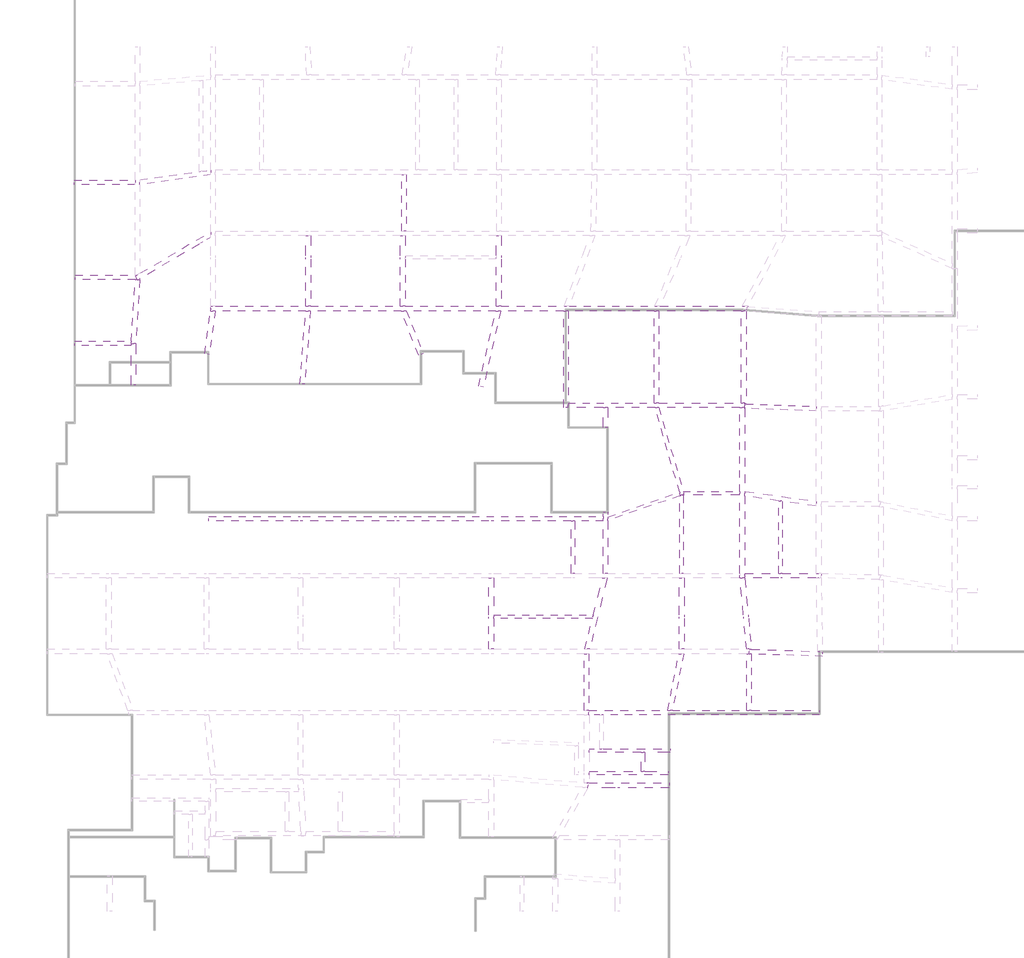
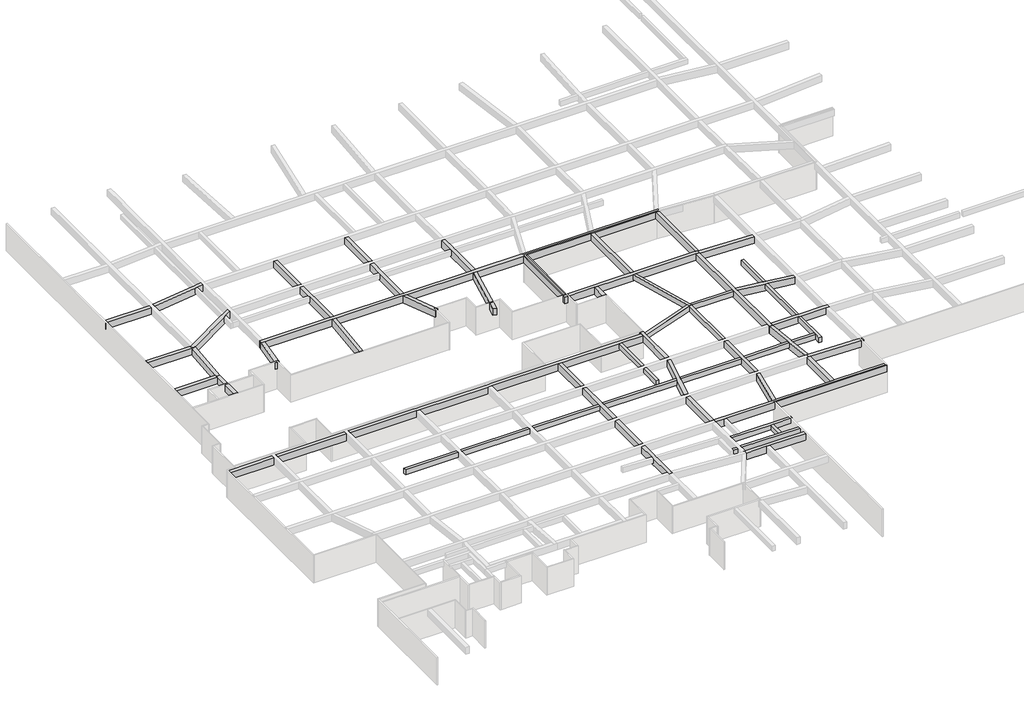
# One storey, part 7 of 16: 47 beams.
"""IFC4 building model written with IfcOpenShell, lengths in millimetres."""

from ifc_helpers import new_model, si_unit, frame, origin, place, context, project, spatial, polyline, outline, extrude, faceted_brep, element, save

model = new_model("IFC4")

# Units and contexts
model_context = context("Model", 3, world=origin())
ifc_project = project(units=[si_unit("LENGTHUNIT", "METRE", prefix="MILLI")], contexts=[model_context])

# Site, building, storey
site = spatial("IfcSite", under=ifc_project)
building = spatial("IfcBuilding", under=site)
storey = spatial("IfcBuildingStorey", under=building, Name="户型图", Elevation=0.0)

# Beams
placement = place(None, origin())
element("IfcBeam", 1, ObjectType="混凝土 - 矩形梁 : KL_beam", at=placement, inside=storey, context=model_context, shape_type="Brep", body=[
    faceted_brep([(78176.3134091, 116076.7662248, 3300.0), (78176.3134091, 115889.7208044, 3300.0), (78176.3134091, 115676.7662248, 3300.0), (78551.9803713, 115676.7662248, 3300.0), (86260.0613272, 115676.7662248, 3300.0), (86661.2679399, 115676.7662248, 3300.0), (94380.6776719, 115676.7662248, 3300.0), (94811.3414742, 115676.7662248, 3300.0), (102431.6143421, 115676.7662248, 3300.0), (102841.8811164, 115676.7662248, 3300.0), (108192.7086168, 115676.7662248, 3300.0), (108592.7086168, 115676.7662248, 3300.0), (115895.8554474, 115676.7662248, 3300.0), (116295.8554474, 115676.7662248, 3300.0), (123316.4637871, 115676.7662248, 3300.0), (123636.1686236, 115676.7662248, 3300.0), (123716.4637871, 115826.5354155, 3300.0), (123838.7967449, 116054.7148883, 3300.0), (123850.6190407, 116076.7662248, 3300.0), (123396.7589506, 116076.7662248, 3300.0), (116398.0224861, 116076.7662248, 3300.0), (115963.4783352, 116076.7662248, 3300.0), (108678.3382182, 116076.7662248, 3300.0), (108252.6671092, 116076.7662248, 3300.0), (102882.3515287, 116076.7662248, 3300.0), (102482.3515287, 116076.7662248, 3300.0), (94716.2109037, 116076.7662248, 3300.0), (94316.2109037, 116076.7662248, 3300.0), (86676.2109037, 116076.7662248, 3300.0), (86276.2109037, 116076.7662248, 3300.0), (78576.3134091, 116076.7662248, 3300.0), (78176.3134091, 115676.7662248, 2500.0), (78551.9803713, 115676.7662248, 2500.0), (86260.0613272, 115676.7662248, 2500.0), (86661.2679399, 115676.7662248, 2500.0), (94380.6776719, 115676.7662248, 2500.0), (94811.3414742, 115676.7662248, 2500.0), (102431.6143421, 115676.7662248, 2500.0), (102841.8811164, 115676.7662248, 2500.0), (108192.7086168, 115676.7662248, 2500.0), (108592.7086168, 115676.7662248, 2500.0), (115895.8554474, 115676.7662248, 2500.0), (116295.8554474, 115676.7662248, 2500.0), (123316.4637871, 115676.7662248, 2500.0), (123636.1686236, 115676.7662248, 2500.0), (78176.3134091, 115889.7208044, 2500.0), (78176.3134091, 116076.7662248, 2500.0), (78576.3134091, 116076.7662248, 2500.0), (86276.2109037, 116076.7662248, 2500.0), (86676.2109037, 116076.7662248, 2500.0), (94316.2109037, 116076.7662248, 2500.0), (94716.2109037, 116076.7662248, 2500.0), (102482.3515287, 116076.7662248, 2500.0), (102882.3515287, 116076.7662248, 2500.0), (108252.6671092, 116076.7662248, 2500.0), (108678.3382182, 116076.7662248, 2500.0), (115963.4783352, 116076.7662248, 2500.0), (116398.0224861, 116076.7662248, 2500.0), (123396.7589506, 116076.7662248, 2500.0), (123850.6190407, 116076.7662248, 2500.0), (123838.7967449, 116054.7148883, 2500.0), (123716.4637871, 115826.5354155, 2500.0)], [[[0, 1, 2, 3, 4, 5, 6, 7, 8, 9, 10, 11, 12, 13, 14, 15, 16, 17, 18, 19, 20, 21, 22, 23, 24, 25, 26, 27, 28, 29, 30]], [[2, 31, 32, 33, 34, 35, 36, 37, 38, 39, 40, 41, 42, 43, 44, 15, 14, 13, 12, 11, 10, 9, 8, 7, 6, 5, 4, 3]], [[31, 45, 46, 47, 48, 49, 50, 51, 52, 53, 54, 55, 56, 57, 58, 59, 60, 61, 44, 43, 42, 41, 40, 39, 38, 37, 36, 35, 34, 33, 32]], [[46, 0, 30, 29, 28, 27, 26, 25, 24, 23, 22, 21, 20, 19, 18, 59, 58, 57, 56, 55, 54, 53, 52, 51, 50, 49, 48, 47]], [[2, 1, 0, 46, 45, 31]], [[18, 17, 16, 15, 44, 61, 60, 59]]]),
])
element("IfcBeam", 2, ObjectType="混凝土 - 矩形梁 : KL_beam", at=placement, inside=storey, context=model_context, shape_type="SweptSolid", body=[
    extrude(outline(polyline([(78070.7151318, 111977.3325661), (77674.0575313, 112028.9343875), (78176.3134091, 115889.7208044), (78176.3134091, 115676.7662248), (78551.9803713, 115676.7662248), (78070.7151318, 111977.3325661)])), frame((0.0, 0.0, 2500.0), z_axis=(0.0, 0.0, 1.0), x_axis=(1.0, 0.0, 0.0)), (0.0, 0.0, 1.0), 800.0),
])
element("IfcBeam", 3, ObjectType="混凝土 - 矩形梁 : KL_beam", at=placement, inside=storey, context=model_context, shape_type="Brep", body=[
    faceted_brep([(86276.2109037, 116076.7662248, 3300.0), (86676.2109037, 116076.7662248, 3300.0), (86676.2109037, 120066.4564837, 3300.0), (86676.2109037, 120366.4564837, 3300.0), (86676.2109037, 122085.5220623, 3300.0), (86276.2109037, 122085.5220623, 3300.0), (86276.2109037, 120366.4564837, 3300.0), (86276.2109037, 120066.4564837, 3300.0), (86676.2109037, 116076.7662248, 2500.0), (86676.2109037, 122085.5220623, 2500.0), (86276.2109037, 116076.7662248, 2500.0), (86276.2109037, 122085.5220623, 2500.0)], [[[0, 1, 2, 3, 4, 5, 6, 7]], [[1, 8, 9, 4, 3, 2]], [[8, 10, 11, 9]], [[10, 0, 7, 6, 5, 11]], [[1, 0, 10, 8]], [[5, 4, 9, 11]]]),
    faceted_brep([(86276.2109037, 127293.5189202, 3300.0), (86676.2109037, 127293.5189202, 3300.0), (86676.2109037, 127293.5189202, 2500.0), (86276.2109037, 127293.5189202, 2500.0), (86676.2109037, 122485.5220623, 3300.0), (86276.2109037, 122485.5220623, 3300.0), (86276.2109037, 122485.5220623, 2500.0), (86676.2109037, 122485.5220623, 2500.0)], [[[0, 1, 2, 3]], [[4, 5, 6, 7]], [[1, 0, 5, 4]], [[2, 1, 4, 7]], [[3, 2, 7, 6]], [[0, 3, 6, 5]]]),
])
element("IfcBeam", 4, ObjectType="混凝土 - 矩形梁 : KL_beam", at=placement, inside=storey, context=model_context, shape_type="Brep", body=[
    faceted_brep([(102882.3515287, 122085.5220623, 3300.0), (102482.3515287, 122085.5220623, 3300.0), (102482.3515287, 120366.4564837, 3300.0), (102482.3515287, 120066.4564837, 3300.0), (102482.3515287, 116076.7662248, 3300.0), (102882.3515287, 116076.7662248, 3300.0), (102882.3515287, 120066.4564837, 3300.0), (102882.3515287, 120366.4564837, 3300.0), (102882.3515287, 122085.5220623, 2500.0), (102882.3515287, 116076.7662248, 2500.0), (102482.3515287, 122085.5220623, 2500.0), (102482.3515287, 116076.7662248, 2500.0)], [[[0, 1, 2, 3, 4, 5, 6, 7]], [[8, 0, 7, 6, 5, 9]], [[10, 8, 9, 11]], [[1, 10, 11, 4, 3, 2]], [[1, 0, 8, 10]], [[5, 4, 11, 9]]]),
])
element("IfcBeam", 5, ObjectType="混凝土 - 矩形梁 : KL_beam", at=placement, inside=storey, context=model_context, shape_type="Brep", body=[
    faceted_brep([(94716.2109037, 122085.5220623, 3300.0), (94316.2109037, 122085.5220623, 3300.0), (94316.2109037, 120366.4564837, 3300.0), (94316.2109037, 120066.4564837, 3300.0), (94316.2109037, 116076.7662248, 3300.0), (94716.2109037, 116076.7662248, 3300.0), (94716.2109037, 120066.4564837, 3300.0), (94716.2109037, 120366.4564837, 3300.0), (94316.2109037, 122085.5220623, 2500.0), (94316.2109037, 116076.7662248, 2500.0), (94716.2109037, 122085.5220623, 2500.0), (94716.2109037, 116076.7662248, 2500.0)], [[[0, 1, 2, 3, 4, 5, 6, 7]], [[1, 8, 9, 4, 3, 2]], [[8, 10, 11, 9]], [[10, 0, 7, 6, 5, 11]], [[1, 0, 10, 8]], [[5, 4, 9, 11]]]),
])
element("IfcBeam", 6, ObjectType="混凝土 - 矩形梁 : KL_beam", at=placement, inside=storey, context=model_context, shape_type="SweptSolid", body=[
    extrude(outline(polyline([(94416.2109037, 127293.5189202), (94816.2109037, 127293.5189202), (94816.2109037, 122485.5220623), (94416.2109037, 122485.5220623), (94416.2109037, 127293.5189202)])), frame((0.0, 0.0, 2500.0), z_axis=(0.0, 0.0, 1.0), x_axis=(1.0, 0.0, 0.0)), (0.0, 0.0, 1.0), 800.0),
])
element("IfcBeam", 7, ObjectType="混凝土 - 矩形梁 : KL_beam", at=placement, inside=storey, context=model_context, shape_type="SweptSolid", body=[
    extrude(outline(polyline([(86176.4237609, 109439.3321058), (85777.6267448, 109470.3311365), (86260.0613272, 115676.7662248), (86661.2679399, 115676.7662248), (86176.4237609, 109439.3321058)])), frame((0.0, 0.0, 2500.0), z_axis=(0.0, 0.0, 1.0), x_axis=(1.0, 0.0, 0.0)), (0.0, 0.0, 1.0), 800.0),
])
element("IfcBeam", 8, ObjectType="混凝土 - 矩形梁 : KL_beam", at=placement, inside=storey, context=model_context, shape_type="SweptSolid", body=[
    extrude(outline(polyline([(96258.082923, 112050.7873463), (95886.5634241, 111902.553538), (94380.6776719, 115676.7662248), (94811.3414742, 115676.7662248), (96258.082923, 112050.7873463)])), frame((0.0, 0.0, 2500.0), z_axis=(0.0, 0.0, 1.0), x_axis=(1.0, 0.0, 0.0)), (0.0, 0.0, 1.0), 800.0),
])
element("IfcBeam", 9, ObjectType="混凝土 - 矩形梁 : KL_beam", at=placement, inside=storey, context=model_context, shape_type="SweptSolid", body=[
    extrude(outline(polyline([(101367.3736824, 109210.1671603), (100977.3835345, 109299.0923227), (102431.6143421, 115676.7662248), (102841.8811164, 115676.7662248), (101367.3736824, 109210.1671603)])), frame((0.0, 0.0, 2500.0), z_axis=(0.0, 0.0, 1.0), x_axis=(1.0, 0.0, 0.0)), (0.0, 0.0, 1.0), 800.0),
])
element("IfcBeam", 10, ObjectType="混凝土 - 矩形梁 : KL_beam", at=placement, inside=storey, context=model_context, shape_type="Brep", body=[
    faceted_brep([(108192.7086168, 107454.5259701, 3300.0), (108592.7086168, 107454.5259701, 3300.0), (108592.7086168, 107854.5259701, 3300.0), (108592.7086168, 115676.7662248, 3300.0), (108192.7086168, 115676.7662248, 3300.0), (108192.7086168, 107454.5259701, 2500.0), (108192.7086168, 115676.7662248, 2500.0), (108592.7086168, 107454.5259701, 2500.0), (108592.7086168, 115676.7662248, 2500.0), (108592.7086168, 107854.5259701, 2500.0)], [[[0, 1, 2, 3, 4]], [[5, 0, 4, 6]], [[7, 5, 6, 8, 9]], [[1, 7, 9, 8, 3, 2]], [[4, 3, 8, 6]], [[1, 0, 5, 7]]]),
])
element("IfcBeam", 11, ObjectType="混凝土 - 矩形梁 : KL_beam", at=placement, inside=storey, context=model_context, shape_type="SweptSolid", body=[
    extrude(outline(polyline([(115895.8554474, 115676.7662248), (116295.8554474, 115676.7662248), (116295.8554474, 107854.5259701), (115895.8554474, 107854.5259701), (115895.8554474, 115676.7662248)])), frame((0.0, 0.0, 2500.0), z_axis=(0.0, 0.0, 1.0), x_axis=(1.0, 0.0, 0.0)), (0.0, 0.0, 1.0), 800.0),
])
element("IfcBeam", 12, ObjectType="混凝土 - 矩形梁 : KL_beam", at=placement, inside=storey, context=model_context, shape_type="Brep", body=[
    faceted_brep([(123592.7086168, 107454.5259701, 3300.0), (123592.7086168, 107773.0747643, 3300.0), (123592.7086168, 107854.5259701, 3300.0), (123316.4637871, 107854.5259701, 3300.0), (116295.8554474, 107854.5259701, 3300.0), (115895.8554474, 107854.5259701, 3300.0), (108592.7086168, 107854.5259701, 3300.0), (108592.7086168, 107454.5259701, 3300.0), (111562.3392399, 107454.5259701, 3300.0), (111962.3392399, 107454.5259701, 3300.0), (115997.1596092, 107454.5259701, 3300.0), (116309.2494399, 107454.5259701, 3300.0), (123192.7086168, 107454.5259701, 3300.0), (123592.7086168, 107454.5259701, 2500.0), (108592.7086168, 107454.5259701, 2500.0), (111562.3392399, 107454.5259701, 2500.0), (111962.3392399, 107454.5259701, 2500.0), (123192.7086168, 107454.5259701, 2500.0), (123592.7086168, 107854.5259701, 2500.0), (123592.7086168, 107773.0747643, 2500.0), (108592.7086168, 107854.5259701, 2500.0), (115895.8554474, 107854.5259701, 2500.0), (116295.8554474, 107854.5259701, 2500.0), (123316.4637871, 107854.5259701, 2500.0)], [[[0, 1, 2, 3, 4, 5, 6, 7, 8, 9, 10, 11, 12]], [[13, 0, 12, 11, 10, 9, 8, 7, 14, 15, 16, 17]], [[18, 19, 13, 17, 16, 15, 14, 20, 21, 22, 23]], [[2, 18, 23, 22, 21, 20, 6, 5, 4, 3]], [[7, 6, 20, 14]], [[2, 1, 0, 13, 19, 18]]]),
])
element("IfcBeam", 13, ObjectType="混凝土 - 矩形梁 : KL_beam", at=placement, inside=storey, context=model_context, shape_type="Brep", body=[
    faceted_brep([(123192.7086168, 92954.5259701, 3300.0), (123210.1011003, 92954.5259701, 3300.0), (123592.7086168, 92954.5259701, 3300.0), (123592.7086168, 93163.6175236, 3300.0), (123592.7086168, 93354.5259701, 3300.0), (123592.7086168, 99926.6110603, 3300.0), (123592.7086168, 100330.5420893, 3300.0), (123592.7086168, 107372.8309465, 3300.0), (123592.7086168, 107454.5259701, 3300.0), (123192.7086168, 107454.5259701, 3300.0), (123192.7086168, 100306.6847418, 3300.0), (123192.7086168, 100006.6847418, 3300.0), (123192.7086168, 93354.5259701, 3300.0), (123192.7086168, 92954.5259701, 2500.0), (123192.7086168, 107454.5259701, 2500.0), (123192.7086168, 93354.5259701, 2500.0), (123592.7086168, 92954.5259701, 2500.0), (123210.1011003, 92954.5259701, 2500.0), (123592.7086168, 107454.5259701, 2500.0), (123592.7086168, 107372.8309465, 2500.0), (123592.7086168, 100330.5420893, 2500.0), (123592.7086168, 99926.6110603, 2500.0), (123592.7086168, 93354.5259701, 2500.0), (123592.7086168, 93163.6175236, 2500.0)], [[[0, 1, 2, 3, 4, 5, 6, 7, 8, 9, 10, 11, 12]], [[13, 0, 12, 11, 10, 9, 14, 15]], [[16, 17, 13, 15, 14, 18, 19, 20, 21, 22, 23]], [[2, 16, 23, 22, 21, 20, 19, 18, 8, 7, 6, 5, 4, 3]], [[9, 8, 18, 14]], [[2, 1, 0, 13, 17, 16]]]),
])
element("IfcBeam", 14, ObjectType="混凝土 - 矩形梁 : KL_beam", at=placement, inside=storey, context=model_context, shape_type="Brep", body=[
    faceted_brep([(111562.3392399, 98554.5675961, 3300.0), (111962.3392399, 98554.5675961, 3300.0), (111962.3392399, 98554.5675961, 2500.0), (111562.3392399, 98554.5675961, 2500.0), (111562.3392399, 98206.3384701, 3300.0), (111562.3392399, 97806.3384701, 3300.0), (111562.3392399, 93354.5259701, 3300.0), (111962.3392399, 93354.5259701, 3300.0), (111962.3392399, 97834.463357, 3300.0), (111962.3392399, 98151.7495614, 3300.0), (111962.3392399, 93354.5259701, 2500.0), (111562.3392399, 93354.5259701, 2500.0), (111562.3392399, 97806.3384701, 2500.0), (111562.3392399, 98206.3384701, 2500.0)], [[[0, 1, 2, 3]], [[1, 0, 4, 5, 6, 7, 8, 9]], [[2, 1, 9, 8, 7, 10]], [[3, 2, 10, 11, 12, 13]], [[0, 3, 13, 12, 11, 6, 5, 4]], [[7, 6, 11, 10]]]),
])
element("IfcBeam", 15, ObjectType="混凝土 - 矩形梁 : KL_beam", at=placement, inside=storey, context=model_context, shape_type="SweptSolid", body=[
    extrude(outline(polyline([(111962.3392399, 105755.0675961), (111562.3392399, 105755.0675961), (111562.3392399, 107454.5259701), (111962.3392399, 107454.5259701), (111962.3392399, 105755.0675961)])), frame((0.0, 0.0, 2500.0), z_axis=(0.0, 0.0, 1.0), x_axis=(1.0, 0.0, 0.0)), (0.0, 0.0, 1.0), 800.0),
])
element("IfcBeam", 16, ObjectType="混凝土 - 矩形梁 : KL_beam", at=placement, inside=storey, context=model_context, shape_type="Brep", body=[
    faceted_brep([(130213.9366903, 86678.8974691, 3300.0), (129813.6317555, 86692.8764254, 3300.0), (124164.2446279, 86890.1573711, 3300.0), (123984.5564618, 86896.4322201, 3300.0), (123977.5744358, 86496.4322201, 3300.0), (124181.0654488, 86489.3261573, 3300.0), (130199.9768916, 86279.1411383, 3300.0), (123977.5744358, 86496.4322201, 2500.0), (124181.0654488, 86489.3261573, 2500.0), (130199.9768916, 86279.1411383, 2500.0), (123984.5564618, 86896.4322201, 2500.0), (124164.2446279, 86890.1573711, 2500.0), (129813.6317555, 86692.8764254, 2500.0), (130213.9366903, 86678.8974691, 2500.0)], [[[0, 1, 2, 3, 4, 5, 6]], [[6, 5, 4, 7, 8, 9]], [[9, 8, 7, 10, 11, 12, 13]], [[3, 2, 1, 0, 13, 12, 11, 10]], [[3, 10, 7, 4]], [[0, 6, 9, 13]]]),
])
element("IfcBeam", 17, ObjectType="混凝土 - 矩形梁 : KL_beam", at=placement, inside=storey, context=model_context, shape_type="Brep", body=[
    faceted_brep([(129958.0309855, 81705.2669877, 3300.0), (129958.0309855, 81305.2669877, 3300.0), (129958.0309855, 81305.2669877, 2500.0), (129958.0309855, 81705.2669877, 2500.0), (124181.0654488, 81705.2669877, 3300.0), (123781.0654488, 81705.2669877, 3300.0), (117463.2475338, 81705.2669877, 3300.0), (117055.5101475, 81705.2669877, 3300.0), (110358.0309855, 81705.2669877, 3300.0), (110358.0309855, 81305.2669877, 3300.0), (110366.2091209, 81305.2669877, 3300.0), (111282.2083949, 81305.2669877, 3300.0), (111582.2083949, 81305.2669877, 3300.0), (110358.0309855, 81305.2669877, 2500.0), (110366.2091209, 81305.2669877, 2500.0), (110358.0309855, 81705.2669877, 2500.0), (117055.5101475, 81705.2669877, 2500.0), (117463.2475338, 81705.2669877, 2500.0), (123781.0654488, 81705.2669877, 2500.0), (124181.0654488, 81705.2669877, 2500.0)], [[[0, 1, 2, 3]], [[1, 0, 4, 5, 6, 7, 8, 9, 10, 11, 12]], [[2, 1, 12, 11, 10, 9, 13, 14]], [[3, 2, 14, 13, 15, 16, 17, 18, 19]], [[0, 3, 19, 18, 17, 16, 15, 8, 7, 6, 5, 4]], [[9, 8, 15, 13]]]),
])
element("IfcBeam", 18, ObjectType="混凝土 - 矩形梁 : KL_beam", at=placement, inside=storey, context=model_context, shape_type="Brep", body=[
    faceted_brep([(64281.2023444, 98206.3384701, 3300.0), (64281.2023444, 98206.3384701, 2500.0), (64281.2023444, 97806.3384701, 2500.0), (64281.2023444, 97806.3384701, 3300.0), (69311.5077787, 98206.3384701, 3300.0), (69311.5077787, 97806.3384701, 3300.0), (69311.5077787, 97806.3384701, 2500.0), (69311.5077787, 98206.3384701, 2500.0)], [[[0, 1, 2, 3]], [[4, 5, 6, 7]], [[0, 3, 5, 4]], [[3, 2, 6, 5]], [[2, 1, 7, 6]], [[1, 0, 4, 7]]]),
    faceted_brep([(111562.3392399, 97806.3384701, 3300.0), (111562.3392399, 98206.3384701, 3300.0), (94216.2109037, 98206.3384701, 3300.0), (93816.2109037, 98206.3384701, 3300.0), (86016.2109037, 98206.3384701, 3300.0), (85616.2109037, 98206.3384701, 3300.0), (78016.2109037, 98206.3384701, 3300.0), (78016.2109037, 97806.3384701, 3300.0), (85616.2109037, 97806.3384701, 3300.0), (86016.2109037, 97806.3384701, 3300.0), (93816.2109037, 97806.3384701, 3300.0), (94216.2109037, 97806.3384701, 3300.0), (101845.5053338, 97806.3384701, 3300.0), (102245.5053338, 97806.3384701, 3300.0), (108832.3515287, 97806.3384701, 3300.0), (109132.3515287, 97806.3384701, 3300.0), (111562.3392399, 97806.3384701, 2500.0), (78016.2109037, 97806.3384701, 2500.0), (85616.2109037, 97806.3384701, 2500.0), (86016.2109037, 97806.3384701, 2500.0), (93816.2109037, 97806.3384701, 2500.0), (94216.2109037, 97806.3384701, 2500.0), (101845.5053338, 97806.3384701, 2500.0), (102245.5053338, 97806.3384701, 2500.0), (111562.3392399, 98206.3384701, 2500.0), (78016.2109037, 98206.3384701, 2500.0), (85616.2109037, 98206.3384701, 2500.0), (86016.2109037, 98206.3384701, 2500.0), (93816.2109037, 98206.3384701, 2500.0), (94216.2109037, 98206.3384701, 2500.0)], [[[0, 1, 2, 3, 4, 5, 6, 7, 8, 9, 10, 11, 12, 13, 14, 15]], [[16, 0, 15, 14, 13, 12, 11, 10, 9, 8, 7, 17, 18, 19, 20, 21, 22, 23]], [[24, 16, 23, 22, 21, 20, 19, 18, 17, 25, 26, 27, 28, 29]], [[1, 24, 29, 28, 27, 26, 25, 6, 5, 4, 3, 2]], [[1, 0, 16, 24]], [[7, 6, 25, 17]]]),
    faceted_brep([(77616.2109037, 98206.3384701, 3300.0), (77616.2109037, 97806.3384701, 3300.0), (77616.2109037, 97806.3384701, 2500.0), (77616.2109037, 98206.3384701, 2500.0), (69711.5077787, 98206.3384701, 3300.0), (69711.5077787, 97806.3384701, 3300.0), (69711.5077787, 97806.3384701, 2500.0), (69711.5077787, 98206.3384701, 2500.0)], [[[0, 1, 2, 3]], [[1, 0, 4, 5]], [[2, 1, 5, 6]], [[3, 2, 6, 7]], [[0, 3, 7, 4]], [[5, 4, 7, 6]]]),
])
element("IfcBeam", 19, ObjectType="混凝土 - 矩形梁 : KL_beam", at=placement, inside=storey, context=model_context, shape_type="Brep", body=[
    faceted_brep([(101845.5053338, 75807.4648036, 3300.0), (102245.5053338, 75807.4648036, 3300.0), (102245.5053338, 76191.067841, 3300.0), (102245.5053338, 78907.8745631, 3300.0), (102245.5053338, 79208.0574264, 3300.0), (102245.5053338, 81305.2669877, 3300.0), (101845.5053338, 81305.2669877, 3300.0), (101845.5053338, 79222.0257342, 3300.0), (101845.5053338, 78921.8428709, 3300.0), (101845.5053338, 76207.4648036, 3300.0), (102245.5053338, 75807.4648036, 2500.0), (102245.5053338, 76191.067841, 2500.0), (102245.5053338, 81305.2669877, 2500.0), (101845.5053338, 75807.4648036, 2500.0), (101845.5053338, 76207.4648036, 2500.0), (101845.5053338, 81305.2669877, 2500.0)], [[[0, 1, 2, 3, 4, 5, 6, 7, 8, 9]], [[1, 10, 11, 12, 5, 4, 3, 2]], [[10, 13, 14, 15, 12, 11]], [[13, 0, 9, 8, 7, 6, 15, 14]], [[6, 5, 12, 15]], [[1, 0, 13, 10]]]),
    faceted_brep([(101845.5053338, 97806.3384701, 3300.0), (102245.5053338, 97806.3384701, 3300.0), (102245.5053338, 97806.3384701, 2500.0), (101845.5053338, 97806.3384701, 2500.0), (102245.5053338, 93354.5259701, 3300.0), (101845.5053338, 93354.5259701, 3300.0), (101845.5053338, 93354.5259701, 2500.0), (102245.5053338, 93354.5259701, 2500.0)], [[[0, 1, 2, 3]], [[4, 5, 6, 7]], [[1, 0, 5, 4]], [[2, 1, 4, 7]], [[3, 2, 7, 6]], [[0, 3, 6, 5]]]),
    faceted_brep([(101845.5053338, 92954.5259701, 3300.0), (102245.5053338, 92954.5259701, 3300.0), (102245.5053338, 92954.5259701, 2500.0), (101845.5053338, 92954.5259701, 2500.0), (102245.5053338, 86896.4322201, 3300.0), (101845.5053338, 86896.4322201, 3300.0), (101845.5053338, 86896.4322201, 2500.0), (102245.5053338, 86896.4322201, 2500.0), (101845.5053338, 89798.5734388, 3300.0), (101845.5053338, 89498.5734388, 3300.0), (102245.5053338, 89498.5734388, 3300.0), (102245.5053338, 89798.5734388, 3300.0)], [[[0, 1, 2, 3]], [[4, 5, 6, 7]], [[1, 0, 8, 9, 5, 4, 10, 11]], [[2, 1, 11, 10, 4, 7]], [[3, 2, 7, 6]], [[0, 3, 6, 5, 9, 8]]]),
    faceted_brep([(101845.5053338, 86496.4322201, 3300.0), (102245.5053338, 86496.4322201, 3300.0), (102245.5053338, 86496.4322201, 2500.0), (101845.5053338, 86496.4322201, 2500.0), (102245.5053338, 81705.2669877, 3300.0), (101845.5053338, 81705.2669877, 3300.0), (101845.5053338, 81705.2669877, 2500.0), (102245.5053338, 81705.2669877, 2500.0)], [[[0, 1, 2, 3]], [[4, 5, 6, 7]], [[1, 0, 5, 4]], [[2, 1, 4, 7]], [[3, 2, 7, 6]], [[0, 3, 6, 5]]]),
])
element("IfcBeam", 20, ObjectType="混凝土 - 矩形梁 : KL_beam", at=placement, inside=storey, context=model_context, shape_type="SweptSolid", body=[
    extrude(outline(polyline([(110358.0309855, 81705.2669877), (109958.0309855, 81705.2669877), (109958.0309855, 86496.4322201), (110358.0309855, 86496.4322201), (110358.0309855, 81705.2669877)])), frame((0.0, 0.0, 2500.0), z_axis=(0.0, 0.0, 1.0), x_axis=(1.0, 0.0, 0.0)), (0.0, 0.0, 1.0), 800.0),
])
element("IfcBeam", 21, ObjectType="混凝土 - 矩形梁 : KL_beam", at=placement, inside=storey, context=model_context, shape_type="Brep", body=[
    faceted_brep([(111918.7343757, 92954.5259701, 3300.0), (111506.5768098, 92954.5259701, 3300.0), (110722.5806505, 89798.5734388, 3300.0), (110648.0551798, 89498.5734388, 3300.0), (110001.6358496, 86896.4322201, 3300.0), (110413.7934156, 86896.4322201, 3300.0), (111060.2127458, 89498.5734388, 3300.0), (111134.7382164, 89798.5734388, 3300.0), (111918.7343757, 92954.5259701, 2500.0), (110413.7934156, 86896.4322201, 2500.0), (111506.5768098, 92954.5259701, 2500.0), (110001.6358496, 86896.4322201, 2500.0)], [[[0, 1, 2, 3, 4, 5, 6, 7]], [[8, 0, 7, 6, 5, 9]], [[10, 8, 9, 11]], [[1, 10, 11, 4, 3, 2]], [[1, 0, 8, 10]], [[5, 4, 11, 9]]]),
])
element("IfcBeam", 22, ObjectType="混凝土 - 矩形梁 : KL_beam", at=placement, inside=storey, context=model_context, shape_type="Brep", body=[
    faceted_brep([(118445.8268228, 92954.5259701, 3300.0), (118045.8268228, 92954.5259701, 3300.0), (118045.8268228, 89798.5734388, 3300.0), (118045.8268228, 89498.5734388, 3300.0), (118045.8268228, 86896.4322201, 3300.0), (118445.8268228, 86896.4322201, 3300.0), (118445.8268228, 89498.5734388, 3300.0), (118445.8268228, 89798.5734388, 3300.0), (118045.8268228, 92954.5259701, 2500.0), (118045.8268228, 86896.4322201, 2500.0), (118445.8268228, 92954.5259701, 2500.0), (118445.8268228, 86896.4322201, 2500.0)], [[[0, 1, 2, 3, 4, 5, 6, 7]], [[1, 8, 9, 4, 3, 2]], [[8, 10, 11, 9]], [[10, 0, 7, 6, 5, 11]], [[1, 0, 10, 8]], [[5, 4, 9, 11]]]),
])
element("IfcBeam", 23, ObjectType="混凝土 - 矩形梁 : KL_beam", at=placement, inside=storey, context=model_context, shape_type="Brep", body=[
    faceted_brep([(123592.7086168, 93163.6175236, 3300.0), (123592.7086168, 92954.5259701, 3300.0), (123210.1011003, 92954.5259701, 3300.0), (123497.6203444, 89798.5734388, 3300.0), (123524.9514821, 89498.5734388, 3300.0), (123762.0164154, 86896.4322201, 3300.0), (123984.5564618, 86896.4322201, 3300.0), (124164.2446279, 86890.1573711, 3300.0), (123926.6080321, 89498.5734388, 3300.0), (123899.2768944, 89798.5734388, 3300.0), (123611.7576503, 92954.5259701, 3300.0), (123210.1011003, 92954.5259701, 2500.0), (123762.0164154, 86896.4322201, 2500.0), (123592.7086168, 92954.5259701, 2500.0), (123592.7086168, 93163.6175236, 2500.0), (123611.7576503, 92954.5259701, 2500.0), (124164.2446279, 86890.1573711, 2500.0), (123984.5564618, 86896.4322201, 2500.0)], [[[0, 1, 2, 3, 4, 5, 6, 7, 8, 9, 10]], [[2, 11, 12, 5, 4, 3]], [[13, 14, 15, 16, 17, 12, 11]], [[14, 0, 10, 9, 8, 7, 16, 15]], [[13, 1, 0, 14]], [[1, 13, 11, 2]], [[6, 5, 12, 17]], [[7, 6, 17, 16]]]),
])
element("IfcBeam", 24, ObjectType="混凝土 - 矩形梁 : KL_beam", at=placement, inside=storey, context=model_context, shape_type="Brep", body=[
    faceted_brep([(117180.6372849, 75511.9613974, 3300.0), (117180.6372849, 75111.9613974, 3300.0), (117180.6372849, 75111.9613974, 2500.0), (117180.6372849, 75511.9613974, 2500.0), (110366.2091209, 75511.9613974, 3300.0), (110174.7580431, 75511.9613974, 3300.0), (110307.6727181, 75500.5778263, 3300.0), (110274.3893899, 75111.9613974, 3300.0), (112596.0859037, 75111.9613974, 3300.0), (112996.0859037, 75111.9613974, 3300.0), (110274.3893899, 75111.9613974, 2500.0), (112596.0859037, 75111.9613974, 2500.0), (112996.0859037, 75111.9613974, 2500.0), (110307.6727181, 75500.5778263, 2500.0), (110174.7580431, 75511.9613974, 2500.0), (110366.2091209, 75511.9613974, 2500.0)], [[[0, 1, 2, 3]], [[1, 0, 4, 5, 6, 7, 8, 9]], [[2, 1, 9, 8, 7, 10, 11, 12]], [[3, 2, 12, 11, 10, 13, 14, 15]], [[0, 3, 15, 14, 5, 4]], [[13, 6, 5, 14]], [[6, 13, 10, 7]]]),
])
element("IfcBeam", 25, ObjectType="混凝土 - 矩形梁 : KL_beam", at=placement, inside=storey, context=model_context, shape_type="Brep", body=[
    faceted_brep([(123592.7086168, 100330.5420893, 3300.0), (123592.7086168, 99926.6110603, 3300.0), (126516.2091266, 99515.7398584, 3300.0), (126816.2091266, 99473.577608, 3300.0), (129700.8737087, 99068.1644398, 3300.0), (129700.8737087, 99472.0954688, 3300.0), (126816.2091266, 99877.508637, 3300.0), (126516.2091266, 99919.6708874, 3300.0), (123592.7086168, 99926.6110603, 2500.0), (129700.8737087, 99068.1644398, 2500.0), (123592.7086168, 100330.5420893, 2500.0), (129700.8737087, 99472.0954688, 2500.0)], [[[0, 1, 2, 3, 4, 5, 6, 7]], [[1, 8, 9, 4, 3, 2]], [[8, 10, 11, 9]], [[10, 0, 7, 6, 5, 11]], [[1, 0, 10, 8]], [[5, 4, 9, 11]]]),
])
element("IfcBeam", 26, ObjectType="混凝土 - 矩形梁 : KL_beam", at=placement, inside=storey, context=model_context, shape_type="Brep", body=[
    faceted_brep([(130100.8737087, 92954.5259701, 3300.0), (130100.8737087, 93349.5213837, 3300.0), (130100.8737087, 93354.5259701, 3300.0), (129700.8737087, 93354.5259701, 3300.0), (126816.2091266, 93354.5259701, 3300.0), (126516.2091266, 93354.5259701, 3300.0), (123592.7086168, 93354.5259701, 3300.0), (123592.7086168, 93163.6175236, 3300.0), (123611.7576503, 92954.5259701, 3300.0), (126516.2091266, 92954.5259701, 3300.0), (126816.2091266, 92954.5259701, 3300.0), (129704.3342561, 92954.5259701, 3300.0), (129898.3397115, 92954.5259701, 3300.0), (130100.8737087, 92954.5259701, 2500.0), (123611.7576503, 92954.5259701, 2500.0), (129704.3342561, 92954.5259701, 2500.0), (129898.3397115, 92954.5259701, 2500.0), (130100.8737087, 93354.5259701, 2500.0), (130100.8737087, 93349.5213837, 2500.0), (123592.7086168, 93163.6175236, 2500.0), (123592.7086168, 93354.5259701, 2500.0), (129700.8737087, 93354.5259701, 2500.0)], [[[0, 1, 2, 3, 4, 5, 6, 7, 8, 9, 10, 11, 12]], [[13, 0, 12, 11, 10, 9, 8, 14, 15, 16]], [[17, 18, 13, 16, 15, 14, 19, 20, 21]], [[20, 6, 5, 4, 3, 2, 17, 21]], [[6, 20, 19, 7]], [[8, 7, 19, 14]], [[2, 1, 0, 13, 18, 17]]]),
])
element("IfcBeam", 27, ObjectType="混凝土 - 矩形梁 : KL_beam", at=placement, inside=storey, context=model_context, shape_type="Brep", body=[
    faceted_brep([(123592.7086168, 107773.0747643, 3300.0), (123592.7086168, 107454.5259701, 3300.0), (123592.7086168, 107372.8309465, 3300.0), (129700.8737087, 107159.5291213, 3300.0), (129700.8737087, 107559.7729391, 3300.0), (123716.4637871, 107768.7531385, 3300.0), (123592.7086168, 107372.8309465, 2500.0), (129700.8737087, 107159.5291213, 2500.0), (123592.7086168, 107454.5259701, 2500.0), (123592.7086168, 107773.0747643, 2500.0), (123716.4637871, 107768.7531385, 2500.0), (129700.8737087, 107559.7729391, 2500.0)], [[[0, 1, 2, 3, 4, 5]], [[2, 6, 7, 3]], [[6, 8, 9, 10, 11, 7]], [[9, 0, 5, 4, 11, 10]], [[2, 1, 0, 9, 8, 6]], [[4, 3, 7, 11]]]),
])
element("IfcBeam", 28, ObjectType="混凝土 - 矩形梁 : KL_beam", at=placement, inside=storey, context=model_context, shape_type="Brep", body=[
    faceted_brep([(123636.1686236, 115676.7662248, 3300.0), (123316.4637871, 115676.7662248, 3300.0), (123316.4637871, 107854.5259701, 3300.0), (123592.7086168, 107854.5259701, 3300.0), (123592.7086168, 107773.0747643, 3300.0), (123716.4637871, 107768.7531385, 3300.0), (123716.4637871, 115662.2924828, 3300.0), (123716.4637871, 115826.5354155, 3300.0), (123316.4637871, 115676.7662248, 2500.0), (123316.4637871, 107854.5259701, 2500.0), (123636.1686236, 115676.7662248, 2500.0), (123716.4637871, 115826.5354155, 2500.0), (123716.4637871, 115662.2924828, 2500.0), (123716.4637871, 107768.7531385, 2500.0), (123592.7086168, 107773.0747643, 2500.0), (123592.7086168, 107854.5259701, 2500.0)], [[[0, 1, 2, 3, 4, 5, 6, 7]], [[1, 8, 9, 2]], [[8, 10, 11, 12, 13, 14, 15, 9]], [[11, 7, 6, 5, 13, 12]], [[0, 10, 8, 1]], [[10, 0, 7, 11]], [[15, 3, 2, 9]], [[3, 15, 14, 4]], [[5, 4, 14, 13]]]),
])
element("IfcBeam", 29, ObjectType="混凝土 - 矩形梁 : KL_beam", at=placement, inside=storey, context=model_context, shape_type="Brep", body=[
    faceted_brep([(78176.3134091, 127264.1539482, 3300.0), (78176.3134091, 127667.9134655, 3300.0), (77490.6700269, 127573.6881924, 3300.0), (77190.6700269, 127532.4603724, 3300.0), (72166.4204182, 126841.9975108, 3300.0), (72166.4204182, 126438.2379935, 3300.0), (77190.6700269, 127128.7008551, 3300.0), (77490.6700269, 127169.9286751, 3300.0), (78176.3134091, 127667.9134655, 2500.0), (72166.4204182, 126841.9975108, 2500.0), (78176.3134091, 127264.1539482, 2500.0), (72166.4204182, 126438.2379935, 2500.0)], [[[0, 1, 2, 3, 4, 5, 6, 7]], [[1, 8, 9, 4, 3, 2]], [[8, 10, 11, 9]], [[10, 0, 7, 6, 5, 11]], [[1, 0, 10, 8]], [[5, 4, 9, 11]]]),
])
element("IfcBeam", 30, ObjectType="混凝土 - 矩形梁 : KL_beam", at=placement, inside=storey, context=model_context, shape_type="Brep", body=[
    faceted_brep([(71766.4204182, 118644.3414905, 3300.0), (71950.7657908, 118329.7253879, 3300.0), (71968.6390183, 118299.2217464, 3300.0), (72020.6985666, 118329.7253879, 3300.0), (72159.5260067, 118411.0695912, 3300.0), (77190.6700269, 121359.0055405, 3300.0), (77490.6700269, 121534.7867905, 3300.0), (78176.3134091, 121936.5309598, 3300.0), (78176.3134091, 122400.1381649, 3300.0), (77490.6700269, 121998.3939956, 3300.0), (77190.6700269, 121822.6127456, 3300.0), (72166.4204182, 118878.7164905, 3300.0), (71766.4204182, 118644.3414905, 2500.0), (78176.3134091, 122400.1381649, 2500.0), (72166.4204182, 118878.7164905, 2500.0), (71968.6390183, 118299.2217464, 2500.0), (71950.7657908, 118329.7253879, 2500.0), (78176.3134091, 121936.5309598, 2500.0), (72159.5260067, 118411.0695912, 2500.0), (72020.6985666, 118329.7253879, 2500.0)], [[[0, 1, 2, 3, 4, 5, 6, 7, 8, 9, 10, 11]], [[12, 0, 11, 10, 9, 8, 13, 14]], [[15, 16, 12, 14, 13, 17, 18, 19]], [[2, 15, 19, 18, 17, 7, 6, 5, 4, 3]], [[8, 7, 17, 13]], [[2, 1, 0, 12, 16, 15]]]),
])
element("IfcBeam", 31, ObjectType="混凝土 - 矩形梁 : KL_beam", at=placement, inside=storey, context=model_context, shape_type="Brep", body=[
    faceted_brep([(66666.4204182, 118329.7253879, 3300.0), (66666.4204182, 118729.7253879, 3300.0), (66666.4204182, 118729.7253879, 2500.0), (66666.4204182, 118329.7253879, 2500.0), (71753.7925243, 118329.7253879, 3300.0), (71950.7657908, 118329.7253879, 3300.0), (71766.4204182, 118644.3414905, 3300.0), (71766.4204182, 118729.7253879, 3300.0), (71766.4204182, 118729.7253879, 2500.0), (71766.4204182, 118644.3414905, 2500.0), (71950.7657908, 118329.7253879, 2500.0), (71753.7925243, 118329.7253879, 2500.0)], [[[0, 1, 2, 3]], [[1, 0, 4, 5, 6, 7]], [[2, 1, 7, 8]], [[3, 2, 8, 9, 10, 11]], [[0, 3, 11, 10, 5, 4]], [[7, 6, 9, 8]], [[6, 5, 10, 9]]]),
    faceted_brep([(72154.5424904, 118329.7253879, 3300.0), (72154.5424904, 118329.7253879, 2500.0), (72159.5260067, 118411.0695912, 2500.0), (72159.5260067, 118411.0695912, 3300.0), (72020.6985666, 118329.7253879, 3300.0), (72020.6985666, 118329.7253879, 2500.0)], [[[0, 1, 2, 3]], [[4, 3, 2, 5]], [[4, 0, 3]], [[1, 5, 2]], [[1, 0, 4, 5]]]),
])
element("IfcBeam", 32, ObjectType="混凝土 - 矩形梁 : KL_beam", at=placement, inside=storey, context=model_context, shape_type="SweptSolid", body=[
    extrude(outline(polyline([(66566.4204182, 126412.6325388), (66566.4204182, 126812.6325388), (71766.4204182, 126812.6325388), (71766.4204182, 126412.6325388), (66566.4204182, 126412.6325388)])), frame((0.0, 0.0, 2500.0), z_axis=(0.0, 0.0, 1.0), x_axis=(1.0, 0.0, 0.0)), (0.0, 0.0, 1.0), 800.0),
])
element("IfcBeam", 33, ObjectType="混凝土 - 矩形梁 : KL_beam", at=placement, inside=storey, context=model_context, shape_type="Brep", body=[
    faceted_brep([(71422.2890287, 112918.7091876, 3300.0), (71822.2890287, 112906.4677526, 3300.0), (72154.5424904, 118329.7253879, 3300.0), (72020.6985666, 118329.7253879, 3300.0), (71968.6390183, 118299.2217464, 3300.0), (71950.7657908, 118329.7253879, 3300.0), (71753.7925243, 118329.7253879, 3300.0), (71434.1669565, 113112.5884701, 3300.0), (71422.2890287, 112918.7091876, 2500.0), (71753.7925243, 118329.7253879, 2500.0), (71434.1669565, 113112.5884701, 2500.0), (71822.2890287, 112906.4677526, 2500.0), (71950.7657908, 118329.7253879, 2500.0), (71968.6390183, 118299.2217464, 2500.0), (72020.6985666, 118329.7253879, 2500.0), (72154.5424904, 118329.7253879, 2500.0)], [[[0, 1, 2, 3, 4, 5, 6, 7]], [[8, 0, 7, 6, 9, 10]], [[11, 8, 10, 9, 12, 13, 14, 15]], [[1, 11, 15, 2]], [[13, 4, 3, 14]], [[4, 13, 12, 5]], [[6, 5, 12, 9]], [[3, 2, 15, 14]], [[1, 0, 8, 11]]]),
])
element("IfcBeam", 34, ObjectType="混凝土 - 矩形梁 : KL_beam", at=placement, inside=storey, context=model_context, shape_type="Brep", body=[
    faceted_brep([(71822.2890287, 109354.5572201, 3300.0), (71422.2890287, 109354.5572201, 3300.0), (71422.2890287, 109354.5572201, 2500.0), (71822.2890287, 109354.5572201, 2500.0), (71822.2890287, 112906.4677526, 3300.0), (71422.2890287, 112918.7091876, 3300.0), (71422.2890287, 112712.5884701, 3300.0), (71422.2890287, 112918.7091876, 2500.0), (71422.2890287, 112712.5884701, 2500.0), (71822.2890287, 112906.4677526, 2500.0)], [[[0, 1, 2, 3]], [[1, 0, 4, 5, 6]], [[2, 1, 6, 5, 7, 8]], [[3, 2, 8, 7, 9]], [[0, 3, 9, 4]], [[4, 9, 7, 5]]]),
])
element("IfcBeam", 35, ObjectType="混凝土 - 矩形梁 : KL_beam", at=placement, inside=storey, context=model_context, shape_type="SweptSolid", body=[
    extrude(outline(polyline([(66621.8682613, 112712.5884701), (66621.8682613, 113112.5884701), (71434.1669565, 113112.5884701), (71422.2890287, 112918.7091876), (71422.2890287, 112712.5884701), (66621.8682613, 112712.5884701)])), frame((0.0, 0.0, 2500.0), z_axis=(0.0, 0.0, 1.0), x_axis=(1.0, 0.0, 0.0)), (0.0, 0.0, 1.0), 800.0),
])
element("IfcBeam", 36, ObjectType="混凝土 - 矩形梁 : KL_beam", at=placement, inside=storey, context=model_context, shape_type="SweptSolid", body=[
    extrude(outline(polyline([(118002.4303666, 86496.4322201), (118410.1677529, 86496.4322201), (117463.2475338, 81705.2669877), (117055.5101475, 81705.2669877), (118002.4303666, 86496.4322201)])), frame((0.0, 0.0, 2500.0), z_axis=(0.0, 0.0, 1.0), x_axis=(1.0, 0.0, 0.0)), (0.0, 0.0, 1.0), 800.0),
])
element("IfcBeam", 37, ObjectType="混凝土 - 矩形梁 : KL_beam", at=placement, inside=storey, context=model_context, shape_type="Brep", body=[
    faceted_brep([(124181.0654488, 86489.3261573, 3300.0), (123977.5744358, 86496.4322201, 3300.0), (123798.4579323, 86496.4322201, 3300.0), (123781.0654488, 86496.4322201, 3300.0), (123781.0654488, 81705.2669877, 3300.0), (124181.0654488, 81705.2669877, 3300.0), (123781.0654488, 86496.4322201, 2500.0), (123781.0654488, 81705.2669877, 2500.0), (123977.5744358, 86496.4322201, 2500.0), (124181.0654488, 86489.3261573, 2500.0), (124181.0654488, 81705.2669877, 2500.0), (123798.4579323, 86496.4322201, 2500.0)], [[[0, 1, 2, 3, 4, 5]], [[3, 6, 7, 4]], [[8, 9, 10, 7, 6, 11]], [[9, 0, 5, 10]], [[6, 3, 2, 1, 8, 11]], [[1, 0, 9, 8]], [[5, 4, 7, 10]]]),
])
element("IfcBeam", 38, ObjectType="混凝土 - 矩形梁 : L_beam", at=placement, inside=storey, context=model_context, shape_type="Brep", body=[
    faceted_brep([(118132.7937153, 100006.6847418, 3300.0), (118270.9282141, 100006.6847418, 3300.0), (118395.8268228, 100006.6847418, 3300.0), (118444.883546, 100006.6847418, 3300.0), (118358.8599303, 100306.6847418, 3300.0), (116309.2494399, 107454.5259701, 3300.0), (115997.1596092, 107454.5259701, 3300.0), (118062.4020558, 100252.1696317, 3300.0), (118132.7937153, 100006.6847418, 2700.0), (115997.1596092, 107454.5259701, 2700.0), (118062.4020558, 100252.1696317, 2700.0), (118444.883546, 100006.6847418, 2700.0), (118395.8268228, 100006.6847418, 2700.0), (118270.9282141, 100006.6847418, 2700.0), (116309.2494399, 107454.5259701, 2700.0), (118358.8599303, 100306.6847418, 2700.0)], [[[0, 1, 2, 3, 4, 5, 6, 7]], [[8, 0, 7, 6, 9, 10]], [[11, 12, 13, 8, 10, 9, 14, 15]], [[3, 11, 15, 14, 5, 4]], [[6, 5, 14, 9]], [[3, 2, 1, 0, 8, 13, 12, 11]]]),
])
element("IfcBeam", 39, ObjectType="混凝土 - 矩形梁 : L_beam", at=placement, inside=storey, context=model_context, shape_type="SweptSolid", body=[
    extrude(outline(polyline([(118444.883546, 100006.6847418), (118358.8599303, 100306.6847418), (123192.7086168, 100306.6847418), (123192.7086168, 100006.6847418), (118444.883546, 100006.6847418)])), frame((0.0, 0.0, 2700.0), z_axis=(0.0, 0.0, 1.0), x_axis=(1.0, 0.0, 0.0)), (0.0, 0.0, 1.0), 600.0),
])
element("IfcBeam", 40, ObjectType="混凝土 - 矩形梁 : L_beam", at=placement, inside=storey, context=model_context, shape_type="Brep", body=[
    faceted_brep([(118132.7937153, 100006.6847418, 3300.0), (118062.4020558, 100252.1696317, 3300.0), (111962.3392399, 98151.7495614, 3300.0), (111962.3392399, 97834.463357, 3300.0), (118095.8268228, 99946.3924976, 3300.0), (118270.9282141, 100006.6847418, 3300.0), (118062.4020558, 100252.1696317, 2700.0), (111962.3392399, 98151.7495614, 2700.0), (118132.7937153, 100006.6847418, 2700.0), (118270.9282141, 100006.6847418, 2700.0), (118095.8268228, 99946.3924976, 2700.0), (111962.3392399, 97834.463357, 2700.0)], [[[0, 1, 2, 3, 4, 5]], [[1, 6, 7, 2]], [[6, 8, 9, 10, 11, 7]], [[9, 5, 4, 3, 11, 10]], [[0, 8, 6, 1]], [[8, 0, 5, 9]], [[3, 2, 7, 11]]]),
])
element("IfcBeam", 41, ObjectType="混凝土 - 矩形梁 : L_beam", at=placement, inside=storey, context=model_context, shape_type="SweptSolid", body=[
    extrude(outline(polyline([(118270.9282141, 100006.6847418), (118395.8268228, 100006.6847418), (118395.8268228, 93354.5259701), (118095.8268228, 93354.5259701), (118095.8268228, 99946.3924976), (118270.9282141, 100006.6847418)])), frame((0.0, 0.0, 2700.0), z_axis=(0.0, 0.0, 1.0), x_axis=(1.0, 0.0, 0.0)), (0.0, 0.0, 1.0), 600.0),
])
element("IfcBeam", 42, ObjectType="混凝土 - 矩形梁 : L_beam", at=placement, inside=storey, context=model_context, shape_type="Brep", body=[
    faceted_brep([(126816.2091266, 88827.2862006, 3300.0), (126516.2091266, 88827.2862006, 3300.0), (126516.2091266, 88827.2862006, 2700.0), (126816.2091266, 88827.2862006, 2700.0), (126816.2091266, 92954.5259701, 3300.0), (126516.2091266, 92954.5259701, 3300.0), (126516.2091266, 89798.5734388, 3300.0), (126516.2091266, 89498.5734388, 3300.0), (126516.2091266, 92954.5259701, 2700.0), (126516.2091266, 89798.5734388, 2700.0), (126516.2091266, 89498.5734388, 2700.0), (126816.2091266, 92954.5259701, 2700.0)], [[[0, 1, 2, 3]], [[1, 0, 4, 5, 6, 7]], [[2, 1, 7, 6, 5, 8, 9, 10]], [[3, 2, 10, 9, 8, 11]], [[0, 3, 11, 4]], [[5, 4, 11, 8]]]),
    faceted_brep([(126816.2091266, 104238.2862006, 3300.0), (126816.2091266, 104238.2862006, 2700.0), (126516.2091266, 104238.2862006, 2700.0), (126516.2091266, 104238.2862006, 3300.0), (126816.2091266, 99877.508637, 3300.0), (126516.2091266, 99919.6708874, 3300.0), (126516.2091266, 99919.6708874, 2700.0), (126816.2091266, 99877.508637, 2700.0)], [[[0, 1, 2, 3]], [[4, 5, 6, 7]], [[0, 3, 5, 4]], [[3, 2, 6, 5]], [[2, 1, 7, 6]], [[1, 0, 4, 7]]]),
    faceted_brep([(126516.2091266, 99515.7398584, 3300.0), (126816.2091266, 99473.577608, 3300.0), (126816.2091266, 99473.577608, 2700.0), (126516.2091266, 99515.7398584, 2700.0), (126816.2091266, 93354.5259701, 3300.0), (126516.2091266, 93354.5259701, 3300.0), (126516.2091266, 93354.5259701, 2700.0), (126816.2091266, 93354.5259701, 2700.0)], [[[0, 1, 2, 3]], [[4, 5, 6, 7]], [[1, 0, 5, 4]], [[0, 3, 6, 5]], [[3, 2, 7, 6]], [[2, 1, 4, 7]]]),
])
element("IfcBeam", 43, ObjectType="混凝土 - 矩形梁 : L_beam", at=placement, inside=storey, context=model_context, shape_type="SweptSolid", body=[
    extrude(outline(polyline([(79562.7315977, 89498.5734388), (79562.7315977, 89798.5734388), (85616.2109037, 89798.5734388), (85616.2109037, 89498.5734388), (79562.7315977, 89498.5734388)])), frame((0.0, 0.0, 2700.0), z_axis=(0.0, 0.0, 1.0), x_axis=(1.0, 0.0, 0.0)), (0.0, 0.0, 1.0), 600.0),
    extrude(outline(polyline([(86016.2109037, 89498.5734388), (86016.2109037, 89798.5734388), (93816.2109037, 89798.5734388), (93816.2109037, 89498.5734388), (86016.2109037, 89498.5734388)])), frame((0.0, 0.0, 2700.0), z_axis=(0.0, 0.0, 1.0), x_axis=(1.0, 0.0, 0.0)), (0.0, 0.0, 1.0), 600.0),
    extrude(outline(polyline([(126516.2091266, 89798.5734388), (126516.2091266, 89498.5734388), (123926.6080321, 89498.5734388), (123899.2768944, 89798.5734388), (126516.2091266, 89798.5734388)])), frame((0.0, 0.0, 2700.0), z_axis=(0.0, 0.0, 1.0), x_axis=(1.0, 0.0, 0.0)), (0.0, 0.0, 1.0), 600.0),
    extrude(outline(polyline([(94216.2109037, 89498.5734388), (94216.2109037, 89798.5734388), (101845.5053338, 89798.5734388), (101845.5053338, 89498.5734388), (94216.2109037, 89498.5734388)])), frame((0.0, 0.0, 2700.0), z_axis=(0.0, 0.0, 1.0), x_axis=(1.0, 0.0, 0.0)), (0.0, 0.0, 1.0), 600.0),
    extrude(outline(polyline([(102245.5053338, 89498.5734388), (102245.5053338, 89798.5734388), (110722.5806505, 89798.5734388), (110648.0551798, 89498.5734388), (102245.5053338, 89498.5734388)])), frame((0.0, 0.0, 2700.0), z_axis=(0.0, 0.0, 1.0), x_axis=(1.0, 0.0, 0.0)), (0.0, 0.0, 1.0), 600.0),
    extrude(outline(polyline([(111060.2127458, 89498.5734388), (111134.7382164, 89798.5734388), (118045.8268228, 89798.5734388), (118045.8268228, 89498.5734388), (111060.2127458, 89498.5734388)])), frame((0.0, 0.0, 2700.0), z_axis=(0.0, 0.0, 1.0), x_axis=(1.0, 0.0, 0.0)), (0.0, 0.0, 1.0), 600.0),
    extrude(outline(polyline([(118445.8268228, 89498.5734388), (118445.8268228, 89798.5734388), (123497.6203444, 89798.5734388), (123524.9514821, 89498.5734388), (118445.8268228, 89498.5734388)])), frame((0.0, 0.0, 2700.0), z_axis=(0.0, 0.0, 1.0), x_axis=(1.0, 0.0, 0.0)), (0.0, 0.0, 1.0), 600.0),
])
element("IfcBeam", 44, ObjectType="混凝土 - 矩形梁 : L_beam", at=placement, inside=storey, context=model_context, shape_type="Brep", body=[
    faceted_brep([(117097.2170869, 76505.2063644, 3300.0), (117097.2170869, 76205.2063644, 3300.0), (117097.2170869, 76205.2063644, 2700.0), (117097.2170869, 76505.2063644, 2700.0), (115122.4394324, 76505.2063644, 3300.0), (114822.4394324, 76505.2063644, 3300.0), (110366.2091209, 76505.2063644, 3300.0), (110366.2091209, 76205.2063644, 3300.0), (110366.2091209, 76205.2063644, 2700.0), (110366.2091209, 76505.2063644, 2700.0), (114822.4394324, 76505.2063644, 2700.0), (115122.4394324, 76505.2063644, 2700.0)], [[[0, 1, 2, 3]], [[1, 0, 4, 5, 6, 7]], [[2, 1, 7, 8]], [[3, 2, 8, 9, 10, 11]], [[0, 3, 11, 10, 9, 6, 5, 4]], [[7, 6, 9, 8]]]),
    faceted_brep([(109442.9464525, 76205.2063644, 3300.0), (109442.9464525, 76505.2063644, 3300.0), (109442.9464525, 76505.2063644, 2700.0), (109442.9464525, 76205.2063644, 2700.0), (109966.2091209, 76505.2063644, 3300.0), (109966.2091209, 76205.2063644, 3300.0), (109966.2091209, 76205.2063644, 2700.0), (109966.2091209, 76505.2063644, 2700.0)], [[[0, 1, 2, 3]], [[4, 5, 6, 7]], [[1, 0, 5, 4]], [[0, 3, 6, 5]], [[3, 2, 7, 6]], [[2, 1, 4, 7]]]),
])
element("IfcBeam", 45, ObjectType="混凝土 - 矩形梁 : L_beam", at=placement, inside=storey, context=model_context, shape_type="SweptSolid", body=[
    extrude(outline(polyline([(109132.3515287, 90449.0559544), (108832.3515287, 90449.0559544), (108832.3515287, 92954.5259701), (109132.3515287, 92954.5259701), (109132.3515287, 90449.0559544)])), frame((0.0, 0.0, 2700.0), z_axis=(0.0, 0.0, 1.0), x_axis=(1.0, 0.0, 0.0)), (0.0, 0.0, 1.0), 600.0),
    extrude(outline(polyline([(108832.3515287, 97806.3384701), (109132.3515287, 97806.3384701), (109132.3515287, 93354.5259701), (108832.3515287, 93354.5259701), (108832.3515287, 97806.3384701)])), frame((0.0, 0.0, 2700.0), z_axis=(0.0, 0.0, 1.0), x_axis=(1.0, 0.0, 0.0)), (0.0, 0.0, 1.0), 600.0),
])
element("IfcBeam", 46, ObjectType="混凝土 - 矩形梁 : L_beam", at=placement, inside=storey, context=model_context, shape_type="Brep", body=[
    faceted_brep([(117253.6939224, 78117.2851311, 3300.0), (117253.6939224, 78117.2851311, 2700.0), (117253.6939224, 78417.2851311, 2700.0), (117253.6939224, 78417.2851311, 3300.0), (111582.2083949, 78417.2851311, 3300.0), (111282.2083949, 78417.2851311, 3300.0), (110366.2091209, 78417.2851311, 3300.0), (110366.2091209, 78117.2851311, 3300.0), (114822.4394324, 78117.2851311, 3300.0), (115122.4394324, 78117.2851311, 3300.0), (111582.2083949, 78417.2851311, 2700.0), (111282.2083949, 78417.2851311, 2700.0), (110366.2091209, 78417.2851311, 2700.0), (115122.4394324, 78117.2851311, 2700.0), (114822.4394324, 78117.2851311, 2700.0), (110366.2091209, 78117.2851311, 2700.0)], [[[0, 1, 2, 3]], [[0, 3, 4, 5, 6, 7, 8, 9]], [[3, 2, 10, 11, 12, 6, 5, 4]], [[2, 1, 13, 14, 15, 12, 11, 10]], [[1, 0, 9, 8, 7, 15, 14, 13]], [[7, 6, 12, 15]]]),
])
element("IfcBeam", 47, ObjectType="混凝土 - 矩形梁 : L_beam", at=placement, inside=storey, context=model_context, shape_type="SweptSolid", body=[
    extrude(outline(polyline([(115122.4394324, 76505.2063644), (114822.4394324, 76505.2063644), (114822.4394324, 78117.2851311), (115122.4394324, 78117.2851311), (115122.4394324, 76505.2063644)])), frame((0.0, 0.0, 2700.0), z_axis=(0.0, 0.0, 1.0), x_axis=(1.0, 0.0, 0.0)), (0.0, 0.0, 1.0), 600.0),
])

save(model, "model.ifc")

# Revit data of these elements
# Type "混凝土 - 矩形梁 : KL_beam"
#   Length [instance default] = 1524 mm
#   b = 400 mm
#   h = 800 mm
#   Structural Material [instance default] = 混凝土 - 现场浇注混凝土
#   Assembly Code = ""
# Type "混凝土 - 矩形梁 : L_beam"
#   Length [instance default] = 1524 mm
#   b = 300 mm
#   h = 600 mm
#   Structural Material [instance default] = none
#   Assembly Code = ""
# Elements 1, 2, 3, 4, 5, 6, 7, 8, 9, 10, 11, 12, 13, 14, 15, 16, 17, 18, 19, 20, 21, 22, 23, 24, 25, 26, 27, 28, 29, 30, 31, 32, 33, 34, 35, 36, 37 (IfcBeam, "混凝土 - 矩形梁 : KL_beam")
#   Comments = ""
#   Structural Material = none
#   Phase Created = 新构造
# Elements 38, 39, 40, 41, 42, 43, 44, 45, 46, 47 (IfcBeam, "混凝土 - 矩形梁 : L_beam")
#   Comments = ""
#   Structural Material = none
#   Phase Created = 新构造
# Materials
#   "混凝土 - 现场浇注混凝土": class "混凝土", colour RGB 192 192 192, transparency 0
